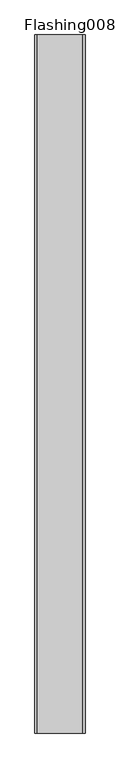
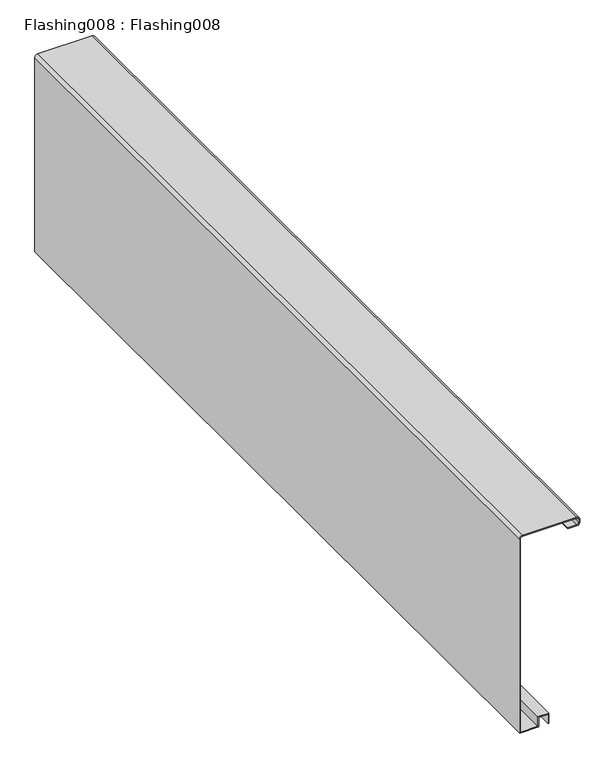
"""IFC4 building model written with IfcOpenShell, lengths in millimetres: proxy geometry, Flashing008 : Flashing008."""

import ifcopenshell
import ifcopenshell.guid

model = None  # the IFC model being written
_history = None  # IfcOwnerHistory: only IFC2X3 demands one
_inside = {}  # id of a spatial element -> (the spatial element, [elements in it])
_under = {}  # id of a project, library or spatial element -> (it, [spatial elements below it])
_declared = {}  # id of a project -> (the project, [libraries it declares])
_typed = {}  # id of a type object -> (the type object, [elements of that type])
_made_of = {}  # id of a material, layer set ... -> (it, [elements and type objects made of it])


def new_model(schema):
    """Start an empty IFC model of exactly this schema.

    Asked for "IFC4X3", IfcOpenShell would pick the latest addendum, in which some entities
    have other attributes; the version numbers below select the first issue.
    IFC2X3 requires an IfcOwnerHistory on every rooted entity: one is made here for all.
    """
    global model, _history
    if schema == "IFC4X3":
        model = ifcopenshell.file(schema_version=(4, 3, 0, 0))
    else:
        model = ifcopenshell.file(schema=schema)
    _inside.clear()
    _under.clear()
    _declared.clear()
    _typed.clear()
    _made_of.clear()
    _history = None
    if model.schema == "IFC2X3":
        org = make("IfcOrganization", Name="unknown")
        user = make(
            "IfcPersonAndOrganization",
            ThePerson=make("IfcPerson", FamilyName="unknown"),
            TheOrganization=org,
        )
        app = make(
            "IfcApplication",
            ApplicationDeveloper=org,
            Version="unknown",
            ApplicationFullName="unknown",
            ApplicationIdentifier="unknown",
        )
        _history = make(
            "IfcOwnerHistory",
            OwningUser=user,
            OwningApplication=app,
            ChangeAction="ADDED",
            CreationDate=0,
        )
    return model


def make(cls, **values):
    """One entity of the class cls with the attributes given. An attribute that is None is left unset."""
    return model.create_entity(
        cls, **{name: value for name, value in values.items() if value is not None}
    )


def rooted(cls, **values):
    """An entity with a GlobalId (a new one), such as an element, a storey or a relation."""
    return make(cls, GlobalId=ifcopenshell.guid.new(), OwnerHistory=_history, **values)


def si_unit(unit_type, name, prefix=None):
    """IfcSIUnit, for example si_unit("LENGTHUNIT", "METRE", prefix="MILLI")."""
    return make("IfcSIUnit", UnitType=unit_type, Prefix=prefix, Name=name)


def assignment(units):
    """IfcUnitAssignment: the units of a project."""
    return None if units is None else make("IfcUnitAssignment", Units=units)


def point(xyz):
    """IfcCartesianPoint."""
    return None if xyz is None else make("IfcCartesianPoint", Coordinates=xyz)


def direction(xyz):
    """IfcDirection."""
    return None if xyz is None else make("IfcDirection", DirectionRatios=xyz)


def frame(location, z_axis=None, x_axis=None):
    """IfcAxis2Placement3D, a coordinate frame: its origin and axes. An axis left out is left unset."""
    return make(
        "IfcAxis2Placement3D",
        Location=point(location),
        Axis=direction(z_axis),
        RefDirection=direction(x_axis),
    )


def frame_2d(location, x_axis=None):
    """IfcAxis2Placement2D, a coordinate frame in the plane: its origin and x axis."""
    return make(
        "IfcAxis2Placement2D", Location=point(location), RefDirection=direction(x_axis)
    )


def origin():
    """The frame at (0, 0, 0) with its axes left unset."""
    return frame((0.0, 0.0, 0.0))


def place(relative_to, where):
    """IfcLocalPlacement: puts the frame where relative to a parent placement (None: the world)."""
    return make(
        "IfcLocalPlacement", PlacementRelTo=relative_to, RelativePlacement=where
    )


def context(
    kind, dimensions, precision=None, world=None, true_north=None, identifier=None
):
    """IfcGeometricRepresentationContext, for example the 3D "Model" context."""
    return make(
        "IfcGeometricRepresentationContext",
        ContextIdentifier=identifier,
        ContextType=kind,
        CoordinateSpaceDimension=dimensions,
        Precision=precision,
        WorldCoordinateSystem=world,
        TrueNorth=true_north,
    )


def project(units=None, contexts=None):
    """IfcProject with its units and contexts."""
    return rooted(
        "IfcProject",
        Name="project",
        RepresentationContexts=contexts,
        UnitsInContext=assignment(units),
    )


def spatial(cls, under=None, at=None, **own):
    """A site, building, storey or space (cls), placed at a placement, below another one or the project."""
    s = rooted(cls, ObjectPlacement=at, **own)
    if under is not None:
        _under.setdefault(under.id(), (under, []))[1].append(s)
    return s


def polyline(points):
    """IfcPolyline through the points."""
    return make("IfcPolyline", Points=[point(p) for p in points])


def circle_curve(where, radius):
    """IfcCircle in the frame where."""
    return make("IfcCircle", Position=where, Radius=radius)


def trimmed(basis, trim1, trim2, sense, master):
    """IfcTrimmedCurve: the piece of a basis curve between two trims."""
    return make(
        "IfcTrimmedCurve",
        BasisCurve=basis,
        Trim1=trim1,
        Trim2=trim2,
        SenseAgreement=sense,
        MasterRepresentation=master,
    )


def segment(curve, same_sense, transition):
    """IfcCompositeCurveSegment."""
    return make(
        "IfcCompositeCurveSegment",
        Transition=transition,
        SameSense=same_sense,
        ParentCurve=curve,
    )


def composite_curve(segments, self_intersect=None):
    """IfcCompositeCurve: segments joined end to end."""
    return make("IfcCompositeCurve", Segments=segments, SelfIntersect=self_intersect)


def outline(outer, holes=None, kind="AREA"):
    """IfcArbitraryClosedProfileDef: a profile drawn as a closed curve; with holes, ...WithVoids."""
    if holes is None:
        return make("IfcArbitraryClosedProfileDef", ProfileType=kind, OuterCurve=outer)
    return make(
        "IfcArbitraryProfileDefWithVoids",
        ProfileType=kind,
        OuterCurve=outer,
        InnerCurves=holes,
    )


def extrude(swept, where, along, depth):
    """IfcExtrudedAreaSolid: the profile swept, set in the frame where, extruded along a direction by depth."""
    return make(
        "IfcExtrudedAreaSolid",
        SweptArea=swept,
        Position=where,
        ExtrudedDirection=direction(along),
        Depth=depth,
    )


def shape(context_of_items, identifier, shape_type, items):
    """IfcShapeRepresentation: the items that make up one representation, for example the "Body"."""
    return make(
        "IfcShapeRepresentation",
        ContextOfItems=context_of_items,
        RepresentationIdentifier=identifier,
        RepresentationType=shape_type,
        Items=items,
    )


def source(mapping_origin, context_of_items, identifier, shape_type, items):
    """IfcRepresentationMap: a shape defined once, which mapped items show again and again."""
    return make(
        "IfcRepresentationMap",
        MappingOrigin=mapping_origin,
        MappedRepresentation=shape(context_of_items, identifier, shape_type, items),
    )


def transform(
    local_origin,
    x_axis=None,
    y_axis=None,
    z_axis=None,
    scale=None,
    scale2=None,
    scale3=None,
    uniform=True,
):
    """IfcCartesianTransformationOperator3D, or its non-uniform kind. x_axis, y_axis, z_axis: its Axis1, 2, 3."""
    if uniform:
        return make(
            "IfcCartesianTransformationOperator3D",
            Axis1=direction(x_axis),
            Axis2=direction(y_axis),
            LocalOrigin=point(local_origin),
            Scale=scale,
            Axis3=direction(z_axis),
        )
    return make(
        "IfcCartesianTransformationOperator3DnonUniform",
        Axis1=direction(x_axis),
        Axis2=direction(y_axis),
        LocalOrigin=point(local_origin),
        Scale=scale,
        Axis3=direction(z_axis),
        Scale2=scale2,
        Scale3=scale3,
    )


def mapped(mapping_source, mapping_target):
    """IfcMappedItem: shows the shape of a source again, moved by a transform."""
    return make(
        "IfcMappedItem", MappingSource=mapping_source, MappingTarget=mapping_target
    )


def made_of(thing, what):
    """Note that an element or type object is made of a material, layer set ...; save() writes the relation."""
    if what is not None:
        _made_of.setdefault(what.id(), (what, []))[1].append(thing)
    return thing


def element(
    cls,
    number,
    at=None,
    inside=None,
    cuts=None,
    type_object=None,
    material=None,
    context=None,
    identifier="Body",
    shape_type=None,
    held_by="IfcProductDefinitionShape",
    body=None,
    shapes=None,
    **own,
):
    """One element of the class cls, such as IfcWall. Its Tag is "e" and its number.

    at: its placement. inside: the storey or other place that contains it. cuts: it is an
    opening in that element (IfcRelVoidsElement). A single representation is given by context,
    identifier, shape_type and body (its items); several are given by shapes. held_by: the class
    of the entity that holds the representations. save() writes the other relations.
    """
    e = rooted(cls, Tag="e%d" % number, ObjectPlacement=at, **own)
    if body is not None:
        shapes = [shape(context, identifier, shape_type, body)]
    if shapes is not None:
        e.Representation = make(held_by, Representations=shapes)
    if inside is not None:
        _inside.setdefault(inside.id(), (inside, []))[1].append(e)
    if cuts is not None:
        rooted(
            "IfcRelVoidsElement", RelatingBuildingElement=cuts, RelatedOpeningElement=e
        )
    if type_object is not None:
        _typed.setdefault(type_object.id(), (type_object, []))[1].append(e)
    return made_of(e, material)


def aggregate(whole, parts):
    """IfcRelAggregates: a whole, such as a stair, and the parts it consists of."""
    return rooted("IfcRelAggregates", RelatingObject=whole, RelatedObjects=parts)


def save(model, path):
    """Write the relations noted so far, then the file.

    IfcRelAggregates (storeys below a building ...), IfcRelContainedInSpatialStructure (elements
    in a storey), IfcRelDefinesByType, IfcRelAssociatesMaterial and IfcRelDeclares: one each for
    every whole, place, type object, material and project.
    """
    for whole, parts in _under.values():
        aggregate(whole, parts)
    for where, things in _inside.values():
        rooted(
            "IfcRelContainedInSpatialStructure",
            RelatedElements=things,
            RelatingStructure=where,
        )
    for kind, things in _typed.values():
        rooted("IfcRelDefinesByType", RelatedObjects=things, RelatingType=kind)
    for what, things in _made_of.values():
        rooted("IfcRelAssociatesMaterial", RelatedObjects=things, RelatingMaterial=what)
    for by, libraries in _declared.values():
        rooted("IfcRelDeclares", RelatingContext=by, RelatedDefinitions=libraries)
    model.write(path)


def flashing008_flashing008_3e815ed5(model_context):
    return source(origin(), model_context, "Body", "SweptSolid", [
        extrude(outline(composite_curve([segment(trimmed(circle_curve(frame_2d((43518.4785937, -6493.7749805)), 5.08), [point((43518.4785937, -6498.8549805))], [point((43523.5585937, -6493.7749805))], True, "CARTESIAN"), True, "CONTINUOUS"), segment(polyline([(43523.5585937, -6493.7749805), (43523.5585937, -6364.4349805)]), True, "CONTINUOUS"), segment(trimmed(circle_curve(frame_2d((43518.4785937, -6364.4349805)), 5.08), [point((43523.5585937, -6364.4349805))], [point((43518.4785937, -6359.3549805))], True, "CARTESIAN"), True, "CONTINUOUS"), segment(polyline([(43518.4785937, -6359.3549805), (43512.0721875, -6359.3549805)]), True, "CONTINUOUS"), segment(trimmed(circle_curve(frame_2d((43512.0721875, -6364.4349805)), 5.08), [point((43512.0721875, -6359.3549805))], [point((43506.9921875, -6364.4349805))], True, "CARTESIAN"), True, "CONTINUOUS"), segment(polyline([(43506.9921875, -6364.4349805), (43506.9921875, -6385.7314453), (43504.9921875, -6385.7314453), (43504.9921875, -6364.4349805)]), True, "CONTINUOUS"), segment(trimmed(circle_curve(frame_2d((43512.0721875, -6364.4349805)), 7.08), [point((43504.9921875, -6364.4349805))], [point((43512.0721875, -6357.3549805))], False, "CARTESIAN"), True, "CONTINUOUS"), segment(polyline([(43512.0721875, -6357.3549805), (43518.4785937, -6357.3549805)]), True, "CONTINUOUS"), segment(trimmed(circle_curve(frame_2d((43518.4785937, -6364.4349805)), 7.08), [point((43518.4785937, -6357.3549805))], [point((43525.5585937, -6364.4349805))], False, "CARTESIAN"), True, "CONTINUOUS"), segment(polyline([(43525.5585937, -6364.4349805), (43525.5585937, -6493.7749805)]), True, "CONTINUOUS"), segment(trimmed(circle_curve(frame_2d((43518.4785937, -6493.7749805)), 7.08), [point((43525.5585937, -6493.7749805))], [point((43518.4785937, -6500.8549805))], False, "CARTESIAN"), True, "CONTINUOUS"), segment(polyline([(43518.4785937, -6500.8549805), (43030.1617235, -6500.8549805), (43030.1617235, -6455.5298267), (43054.2082994, -6455.5298267), (43054.2082994, -6433.1296096), (43030.1617235, -6433.1296096), (43030.1617235, -6431.1296096), (43056.2082994, -6431.1296096), (43056.2082994, -6457.5298267), (43032.1617235, -6457.5298267), (43032.1617235, -6498.8549805), (43518.4785937, -6498.8549805)]), True, "CONTINUOUS")], self_intersect=False)), frame((0.0, 7982.1531721, 0.0), z_axis=(0.0, 1.0, 0.0), x_axis=(0.0, 0.0, 1.0)), (0.0, 0.0, 1.0), 2000.0),
    ])


if __name__ == "__main__":
    model = new_model("IFC4")
    model_context = context("Model", 3, world=origin())
    ifc_project = project(units=[si_unit("LENGTHUNIT", "METRE", prefix="MILLI")], contexts=[model_context])
    site = spatial("IfcSite", under=ifc_project)
    building = spatial("IfcBuilding", under=site)
    placement = place(None, origin())
    flashing008_flashing008_shape = flashing008_flashing008_3e815ed5(model_context)
    element("IfcBuildingElementProxy", 1, Name="Flashing008 : Flashing008", ObjectType="Flashing008 : Flashing008", at=placement, inside=building, context=model_context, shape_type="MappedRepresentation", body=[
        mapped(flashing008_flashing008_shape, transform((0.0, 0.0, 0.0), x_axis=(1.0, 0.0, 0.0), y_axis=(0.0, 1.0, 0.0), z_axis=(0.0, 0.0, 1.0))),
    ])
    save(model, "model.ifc")

# Revit data of these elements
# Type "Flashing008 : Flashing008"
#   NameOverride = "Flashing008"
# Element 1 (IfcBuildingElementProxy, "Flashing008 : Flashing008")
#   Materials on its faces: "BRAKE METAL EAVE TRIM TO MATCH STANDING SEAM COLOR"
# Materials
#   "BRAKE METAL EAVE TRIM TO MATCH STANDING SEAM COLOR": class "Unassigned", colour RGB 128 128 128, transparency 0, Cost = 0
